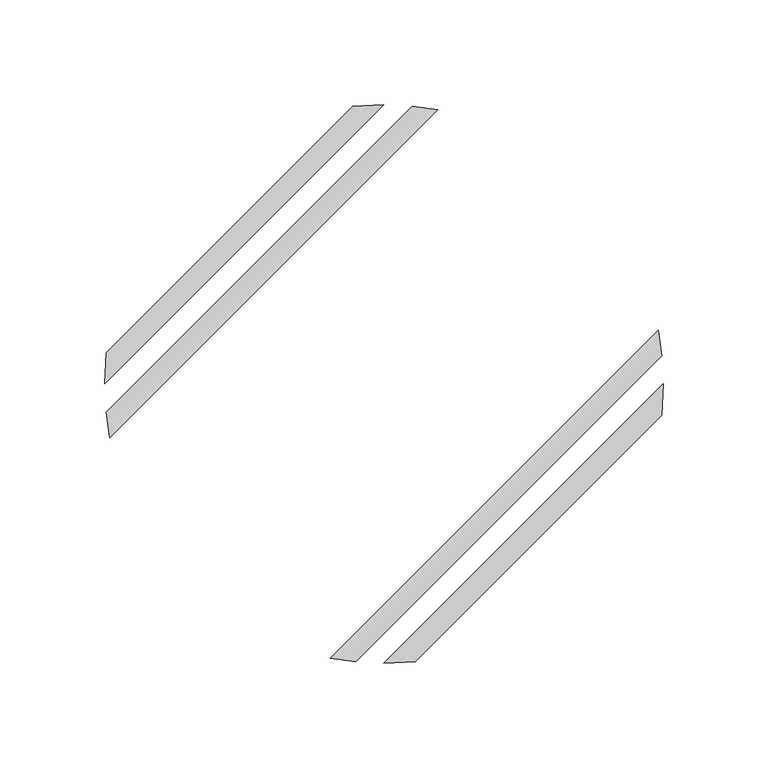
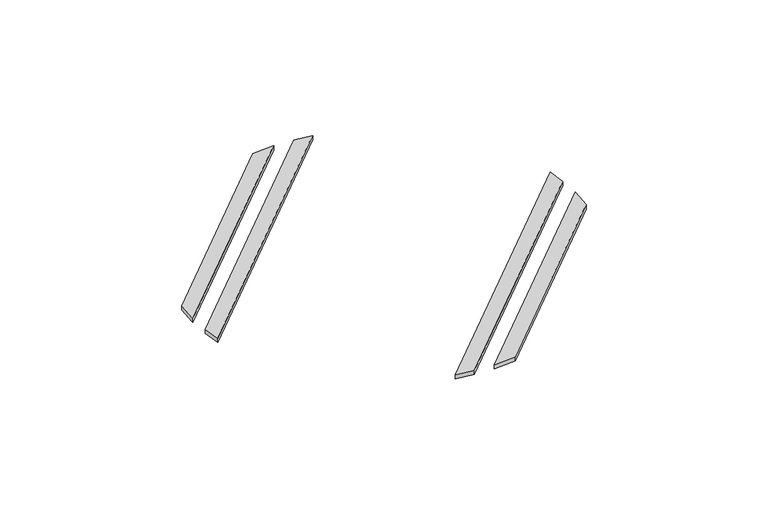
"""IFC4 building model written with IfcOpenShell, lengths in millimetres: proxy geometry, TSP Downlighter in Slab : TSP Downlighter in Slab."""

from ifc_helpers import new_model, si_unit, point, origin, origin_with_axes, origin_2d, place, context, project, spatial, polyline, circle_curve, trimmed, segment, composite_curve, outline, extrude, source, transform, mapped, element, save


def electrical_fixtures_b0e8913b(model_context):
    return source(origin(), model_context, "Body", "SweptSolid", [
        extrude(outline(composite_curve([segment(trimmed(circle_curve(origin_2d(), 133.3333333), [point((-14.987114, 132.4883549))], [point((0.0, 133.3333333))], False, "CARTESIAN"), True, "CONTINUOUS"), segment(polyline([(0.0, 133.3333333), (-133.3333333, 0.0)]), True, "CONTINUOUS"), segment(trimmed(circle_curve(origin_2d(), 133.3333333), [point((-133.3333333, 0.0))], [point((-132.4883549, 14.987114))], False, "CARTESIAN"), True, "CONTINUOUS"), segment(polyline([(-132.4883549, 14.987114), (-14.987114, 132.4883549)]), True, "CONTINUOUS")], self_intersect=False)), origin_with_axes(), (0.0, 0.0, 1.0), 3.0),
        extrude(outline(composite_curve([segment(trimmed(circle_curve(origin_2d(), 133.3333333), [point((14.987114, -132.4883549))], [point((0.0, -133.3333333))], False, "CARTESIAN"), True, "CONTINUOUS"), segment(polyline([(0.0, -133.3333333), (133.3333333, 0.0)]), True, "CONTINUOUS"), segment(trimmed(circle_curve(origin_2d(), 133.3333333), [point((133.3333333, 0.0))], [point((132.4883549, -14.987114))], False, "CARTESIAN"), True, "CONTINUOUS"), segment(polyline([(132.4883549, -14.987114), (14.987114, -132.4883549)]), True, "CONTINUOUS")], self_intersect=False)), origin_with_axes(), (0.0, 0.0, 1.0), 3.0),
        extrude(outline(composite_curve([segment(trimmed(circle_curve(origin_2d(), 133.3333333), [point((13.46091, 132.6521077))], [point((25.7701848, 130.8192469))], False, "CARTESIAN"), True, "CONTINUOUS"), segment(polyline([(25.7701848, 130.8192469), (-130.8192469, -25.7701848)]), True, "CONTINUOUS"), segment(trimmed(circle_curve(origin_2d(), 133.3333333), [point((-130.8192469, -25.7701848))], [point((-132.6521077, -13.46091))], False, "CARTESIAN"), True, "CONTINUOUS"), segment(polyline([(-132.6521077, -13.46091), (13.46091, 132.6521077)]), True, "CONTINUOUS")], self_intersect=False)), origin_with_axes(), (0.0, 0.0, 1.0), 3.0),
        extrude(outline(composite_curve([segment(trimmed(circle_curve(origin_2d(), 133.3333333), [point((-13.46091, -132.6521077))], [point((-25.7701848, -130.8192469))], False, "CARTESIAN"), True, "CONTINUOUS"), segment(polyline([(-25.7701848, -130.8192469), (130.8192469, 25.7701848)]), True, "CONTINUOUS"), segment(trimmed(circle_curve(origin_2d(), 133.3333333), [point((130.8192469, 25.7701848))], [point((132.6521077, 13.46091))], False, "CARTESIAN"), True, "CONTINUOUS"), segment(polyline([(132.6521077, 13.46091), (-13.46091, -132.6521077)]), True, "CONTINUOUS")], self_intersect=False)), origin_with_axes(), (0.0, 0.0, 1.0), 3.0),
    ])


if __name__ == "__main__":
    model = new_model("IFC4")
    model_context = context("Model", 3, world=origin())
    ifc_project = project(units=[si_unit("LENGTHUNIT", "METRE", prefix="MILLI")], contexts=[model_context])
    site = spatial("IfcSite", under=ifc_project)
    building = spatial("IfcBuilding", under=site)
    placement = place(None, origin())
    electrical_fixtures_shape = electrical_fixtures_b0e8913b(model_context)
    element("IfcBuildingElementProxy", 1, Name="TSP Downlighter in Slab : TSP Downlighter in Slab", ObjectType="TSP Downlighter in Slab : TSP Downlighter in Slab", at=placement, inside=building, context=model_context, shape_type="MappedRepresentation", body=[
        mapped(electrical_fixtures_shape, transform((0.0, 0.0, 0.0), x_axis=(1.0, 0.0, 0.0), y_axis=(0.0, 1.0, 0.0), z_axis=(0.0, 0.0, 1.0))),
    ])
    save(model, "model.ifc")

# Revit data of these elements
# Type "TSP Downlighter in Slab : TSP Downlighter in Slab"
#   Model = "TSP_ELEC220DLSLB"
#   Default Elevation = 0
# Element 1 (IfcBuildingElementProxy, "TSP Downlighter in Slab : TSP Downlighter in Slab")
#   Materials on its faces: "Plastic, Opaque Black"
# Materials
#   "Plastic, Opaque Black": class "Plastic", colour RGB 0 0 0, transparency 0.7, Description = "Plastic, generic, opaque black", Cost = 0
